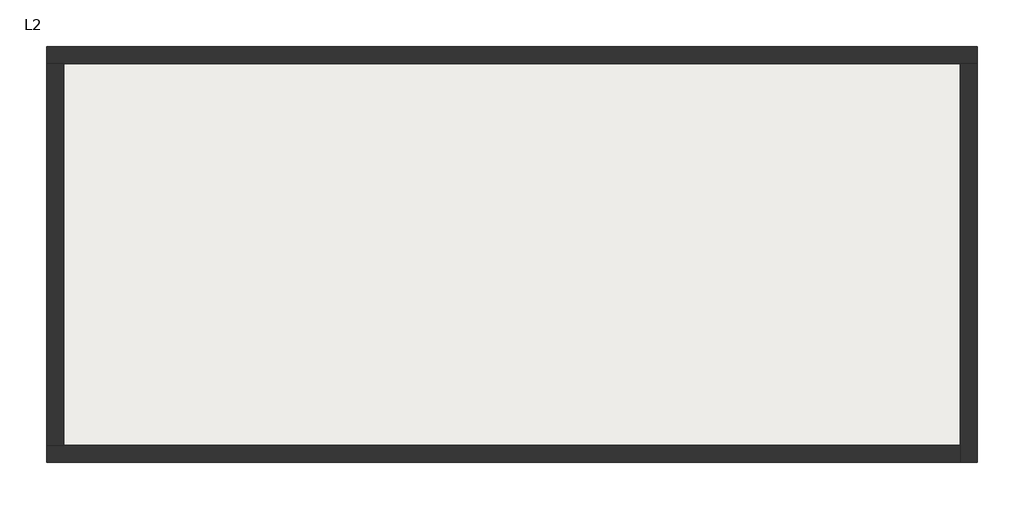
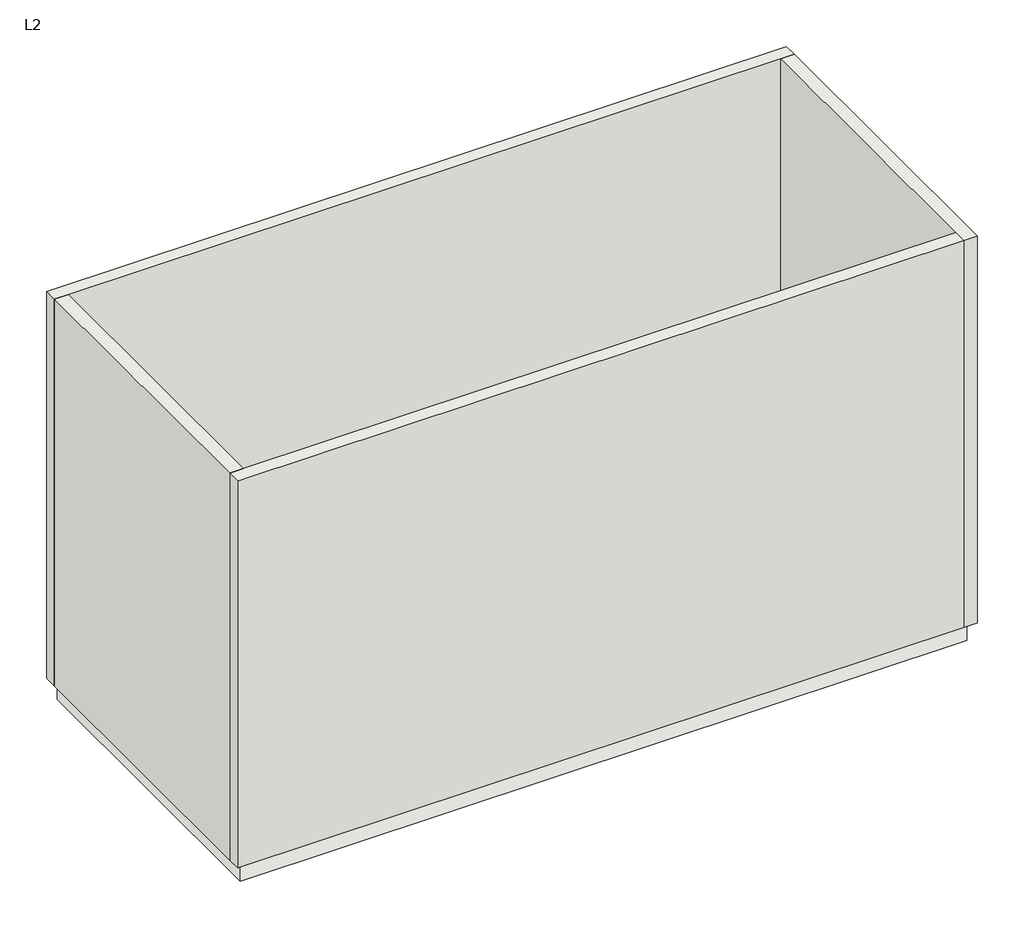
# One storey: 4 walls, 1 slab.
"""IFC4 building model written with IfcOpenShell, lengths in millimetres."""

import ifcopenshell
import ifcopenshell.guid

model = None  # the IFC model being written
_history = None  # IfcOwnerHistory: only IFC2X3 demands one
_inside = {}  # id of a spatial element -> (the spatial element, [elements in it])
_under = {}  # id of a project, library or spatial element -> (it, [spatial elements below it])
_declared = {}  # id of a project -> (the project, [libraries it declares])
_typed = {}  # id of a type object -> (the type object, [elements of that type])
_made_of = {}  # id of a material, layer set ... -> (it, [elements and type objects made of it])


def new_model(schema):
    """Start an empty IFC model of exactly this schema.

    Asked for "IFC4X3", IfcOpenShell would pick the latest addendum, in which some entities
    have other attributes; the version numbers below select the first issue.
    IFC2X3 requires an IfcOwnerHistory on every rooted entity: one is made here for all.
    """
    global model, _history
    if schema == "IFC4X3":
        model = ifcopenshell.file(schema_version=(4, 3, 0, 0))
    else:
        model = ifcopenshell.file(schema=schema)
    _inside.clear()
    _under.clear()
    _declared.clear()
    _typed.clear()
    _made_of.clear()
    _history = None
    if model.schema == "IFC2X3":
        org = make("IfcOrganization", Name="unknown")
        user = make(
            "IfcPersonAndOrganization",
            ThePerson=make("IfcPerson", FamilyName="unknown"),
            TheOrganization=org,
        )
        app = make(
            "IfcApplication",
            ApplicationDeveloper=org,
            Version="unknown",
            ApplicationFullName="unknown",
            ApplicationIdentifier="unknown",
        )
        _history = make(
            "IfcOwnerHistory",
            OwningUser=user,
            OwningApplication=app,
            ChangeAction="ADDED",
            CreationDate=0,
        )
    return model


def make(cls, **values):
    """One entity of the class cls with the attributes given. An attribute that is None is left unset."""
    return model.create_entity(
        cls, **{name: value for name, value in values.items() if value is not None}
    )


def rooted(cls, **values):
    """An entity with a GlobalId (a new one), such as an element, a storey or a relation."""
    return make(cls, GlobalId=ifcopenshell.guid.new(), OwnerHistory=_history, **values)


def si_unit(unit_type, name, prefix=None):
    """IfcSIUnit, for example si_unit("LENGTHUNIT", "METRE", prefix="MILLI")."""
    return make("IfcSIUnit", UnitType=unit_type, Prefix=prefix, Name=name)


def assignment(units):
    """IfcUnitAssignment: the units of a project."""
    return None if units is None else make("IfcUnitAssignment", Units=units)


def point(xyz):
    """IfcCartesianPoint."""
    return None if xyz is None else make("IfcCartesianPoint", Coordinates=xyz)


def direction(xyz):
    """IfcDirection."""
    return None if xyz is None else make("IfcDirection", DirectionRatios=xyz)


def frame(location, z_axis=None, x_axis=None):
    """IfcAxis2Placement3D, a coordinate frame: its origin and axes. An axis left out is left unset."""
    return make(
        "IfcAxis2Placement3D",
        Location=point(location),
        Axis=direction(z_axis),
        RefDirection=direction(x_axis),
    )


def origin():
    """The frame at (0, 0, 0) with its axes left unset."""
    return frame((0.0, 0.0, 0.0))


def place(relative_to, where):
    """IfcLocalPlacement: puts the frame where relative to a parent placement (None: the world)."""
    return make(
        "IfcLocalPlacement", PlacementRelTo=relative_to, RelativePlacement=where
    )


def context(
    kind, dimensions, precision=None, world=None, true_north=None, identifier=None
):
    """IfcGeometricRepresentationContext, for example the 3D "Model" context."""
    return make(
        "IfcGeometricRepresentationContext",
        ContextIdentifier=identifier,
        ContextType=kind,
        CoordinateSpaceDimension=dimensions,
        Precision=precision,
        WorldCoordinateSystem=world,
        TrueNorth=true_north,
    )


def project(units=None, contexts=None):
    """IfcProject with its units and contexts."""
    return rooted(
        "IfcProject",
        Name="project",
        RepresentationContexts=contexts,
        UnitsInContext=assignment(units),
    )


def spatial(cls, under=None, at=None, **own):
    """A site, building, storey or space (cls), placed at a placement, below another one or the project."""
    s = rooted(cls, ObjectPlacement=at, **own)
    if under is not None:
        _under.setdefault(under.id(), (under, []))[1].append(s)
    return s


def polyline(points):
    """IfcPolyline through the points."""
    return make("IfcPolyline", Points=[point(p) for p in points])


def outline(outer, holes=None, kind="AREA"):
    """IfcArbitraryClosedProfileDef: a profile drawn as a closed curve; with holes, ...WithVoids."""
    if holes is None:
        return make("IfcArbitraryClosedProfileDef", ProfileType=kind, OuterCurve=outer)
    return make(
        "IfcArbitraryProfileDefWithVoids",
        ProfileType=kind,
        OuterCurve=outer,
        InnerCurves=holes,
    )


def extrude(swept, where, along, depth):
    """IfcExtrudedAreaSolid: the profile swept, set in the frame where, extruded along a direction by depth."""
    return make(
        "IfcExtrudedAreaSolid",
        SweptArea=swept,
        Position=where,
        ExtrudedDirection=direction(along),
        Depth=depth,
    )


def faces_of(points, faces, orient=None, outer=None):
    """IfcFace entities. A face is a list of loops; a loop is a list of indices into points, from 0.

    orient and outer hold one flag for each loop. By default every Orientation is true, the
    first loop of a face is its IfcFaceOuterBound and the others are IfcFaceBound.
    """
    made = []
    for i, loops in enumerate(faces):
        bounds = []
        for j, loop in enumerate(loops):
            is_outer = j == 0 if outer is None else outer[i][j]
            bounds.append(
                make(
                    "IfcFaceOuterBound" if is_outer else "IfcFaceBound",
                    Bound=make("IfcPolyLoop", Polygon=[points[k] for k in loop]),
                    Orientation=True if orient is None else orient[i][j],
                )
            )
        made.append(make("IfcFace", Bounds=bounds))
    return made


def faceted_brep(points, faces, orient=None, outer=None, voids=None):
    """IfcFacetedBrep: a solid bounded by flat faces; with voids (closed shells), ...WithVoids."""
    shared = [point(p) for p in points]
    hull = make("IfcClosedShell", CfsFaces=faces_of(shared, faces, orient, outer))
    if voids is None:
        return make("IfcFacetedBrep", Outer=hull)
    return make(
        "IfcFacetedBrepWithVoids",
        Outer=hull,
        Voids=[
            make(cls, CfsFaces=faces_of(shared, fs, o, b)) for cls, fs, o, b in voids
        ],
    )


def shape(context_of_items, identifier, shape_type, items):
    """IfcShapeRepresentation: the items that make up one representation, for example the "Body"."""
    return make(
        "IfcShapeRepresentation",
        ContextOfItems=context_of_items,
        RepresentationIdentifier=identifier,
        RepresentationType=shape_type,
        Items=items,
    )


def made_of(thing, what):
    """Note that an element or type object is made of a material, layer set ...; save() writes the relation."""
    if what is not None:
        _made_of.setdefault(what.id(), (what, []))[1].append(thing)
    return thing


def element(
    cls,
    number,
    at=None,
    inside=None,
    cuts=None,
    type_object=None,
    material=None,
    context=None,
    identifier="Body",
    shape_type=None,
    held_by="IfcProductDefinitionShape",
    body=None,
    shapes=None,
    **own,
):
    """One element of the class cls, such as IfcWall. Its Tag is "e" and its number.

    at: its placement. inside: the storey or other place that contains it. cuts: it is an
    opening in that element (IfcRelVoidsElement). A single representation is given by context,
    identifier, shape_type and body (its items); several are given by shapes. held_by: the class
    of the entity that holds the representations. save() writes the other relations.
    """
    e = rooted(cls, Tag="e%d" % number, ObjectPlacement=at, **own)
    if body is not None:
        shapes = [shape(context, identifier, shape_type, body)]
    if shapes is not None:
        e.Representation = make(held_by, Representations=shapes)
    if inside is not None:
        _inside.setdefault(inside.id(), (inside, []))[1].append(e)
    if cuts is not None:
        rooted(
            "IfcRelVoidsElement", RelatingBuildingElement=cuts, RelatedOpeningElement=e
        )
    if type_object is not None:
        _typed.setdefault(type_object.id(), (type_object, []))[1].append(e)
    return made_of(e, material)


def aggregate(whole, parts):
    """IfcRelAggregates: a whole, such as a stair, and the parts it consists of."""
    return rooted("IfcRelAggregates", RelatingObject=whole, RelatedObjects=parts)


def save(model, path):
    """Write the relations noted so far, then the file.

    IfcRelAggregates (storeys below a building ...), IfcRelContainedInSpatialStructure (elements
    in a storey), IfcRelDefinesByType, IfcRelAssociatesMaterial and IfcRelDeclares: one each for
    every whole, place, type object, material and project.
    """
    for whole, parts in _under.values():
        aggregate(whole, parts)
    for where, things in _inside.values():
        rooted(
            "IfcRelContainedInSpatialStructure",
            RelatedElements=things,
            RelatingStructure=where,
        )
    for kind, things in _typed.values():
        rooted("IfcRelDefinesByType", RelatedObjects=things, RelatingType=kind)
    for what, things in _made_of.values():
        rooted("IfcRelAssociatesMaterial", RelatedObjects=things, RelatingMaterial=what)
    for by, libraries in _declared.values():
        rooted("IfcRelDeclares", RelatingContext=by, RelatedDefinitions=libraries)
    model.write(path)


model = new_model("IFC4")

# Units and contexts
model_context = context("Model", 3, world=origin())
ifc_project = project(units=[si_unit("LENGTHUNIT", "METRE", prefix="MILLI")], contexts=[model_context])

# Site, building, storey
site = spatial("IfcSite", under=ifc_project)
building = spatial("IfcBuilding", under=site)
storey = spatial("IfcBuildingStorey", under=building, Name="L2", Elevation=3657.6)

# Slab
placement = place(None, origin())
element("IfcSlab", 1, ObjectType="Generic - 12\"", at=placement, inside=storey, context=model_context, shape_type="SweptSolid", body=[
    extrude(outline(polyline([(23729.8135056, 3861.9420889), (12909.4135056, 3861.9420889), (12909.4135056, 8586.3420889), (23729.8135056, 8586.3420889), (23729.8135056, 3861.9420889)])), frame((0.0, 0.0, 3352.8), z_axis=(0.0, 0.0, 1.0), x_axis=(1.0, 0.0, 0.0)), (0.0, 0.0, 1.0), 304.8),
])

# Walls
element("IfcWall", 2, ObjectType="Generic - 8\"", at=placement, inside=storey, context=model_context, shape_type="Brep", body=[
    faceted_brep([(23831.4135056, 8687.9420889, 3657.6), (12807.8135056, 8687.9420889, 3657.6), (12807.8135056, 8687.9420889, 9753.6), (23831.4135056, 8687.9420889, 9753.6), (23831.4135056, 8484.7420889, 3657.6), (23831.4135056, 8484.7420889, 9753.6), (23628.2135056, 8484.7420889, 9753.6), (13011.0135056, 8484.7420889, 9753.6), (12807.8135056, 8484.7420889, 9753.6), (12807.8135056, 8484.7420889, 3657.6), (13011.0135056, 8484.7420889, 3657.6), (23628.2135056, 8484.7420889, 3657.6)], [[[0, 1, 2, 3]], [[4, 5, 6, 7, 8, 9, 10, 11]], [[1, 0, 4, 11, 10, 9]], [[3, 2, 8, 7, 6, 5]], [[0, 3, 5, 4]], [[2, 1, 9, 8]]]),
])
element("IfcWall", 3, ObjectType="Generic - 8\"", at=placement, inside=storey, context=model_context, shape_type="Brep", body=[
    faceted_brep([(23831.4135056, 3760.3420889, 3657.6), (23831.4135056, 8484.7420889, 3657.6), (23831.4135056, 8484.7420889, 9753.6), (23831.4135056, 3760.3420889, 9753.6), (23628.2135056, 3760.3420889, 3657.6), (23628.2135056, 3760.3420889, 9753.6), (23628.2135056, 3963.5420889, 9753.6), (23628.2135056, 8484.7420889, 9753.6), (23628.2135056, 8484.7420889, 3657.6), (23628.2135056, 3963.5420889, 3657.6)], [[[0, 1, 2, 3]], [[4, 5, 6, 7, 8, 9]], [[1, 0, 4, 9, 8]], [[3, 2, 7, 6, 5]], [[2, 1, 8, 7]], [[0, 3, 5, 4]]]),
])
element("IfcWall", 4, ObjectType="Generic - 8\"", at=placement, inside=storey, context=model_context, shape_type="Brep", body=[
    faceted_brep([(12807.8135056, 3760.3420889, 3657.6), (23628.2135056, 3760.3420889, 3657.6), (23628.2135056, 3760.3420889, 9753.6), (12807.8135056, 3760.3420889, 9753.6), (12807.8135056, 3963.5420889, 3657.6), (12807.8135056, 3963.5420889, 9753.6), (13011.0135056, 3963.5420889, 9753.6), (23628.2135056, 3963.5420889, 9753.6), (23628.2135056, 3963.5420889, 3657.6), (13011.0135056, 3963.5420889, 3657.6)], [[[0, 1, 2, 3]], [[4, 5, 6, 7, 8, 9]], [[1, 0, 4, 9, 8]], [[3, 2, 7, 6, 5]], [[2, 1, 8, 7]], [[0, 3, 5, 4]]]),
])
element("IfcWall", 5, ObjectType="Generic - 8\"", at=placement, inside=storey, context=model_context, shape_type="SweptSolid", body=[
    extrude(outline(polyline([(12807.8135056, 3963.5420889), (12807.8135056, 8484.7420889), (13011.0135056, 8484.7420889), (13011.0135056, 3963.5420889), (12807.8135056, 3963.5420889)])), frame((0.0, 0.0, 3657.6), z_axis=(0.0, 0.0, 1.0), x_axis=(1.0, 0.0, 0.0)), (0.0, 0.0, 1.0), 6096.0),
])

save(model, "model.ifc")

# Revit data of these elements
# Project information
#   Organization Name = "Organization Name"
#   Organization Description = "Organization Description"
#   Building Name = "Building Name"
#   Project Issue Date = "Issue Date"
#   Project Status = "Project Status"
#   Client Name = "Client Name"
#   Project Address = "Enter address here\nAddress Line 2"
#   Project Name = "Project Name"
#   Project Number = "Project Number"
# Type "Generic - 12\""
#   Description = "Generic Floor (Material By Category), 12\" thick"
#   Type Mark = "G01"
#   Function = 0
#   Layers, outside or top first: 1' - 0" no material (function 1)
# Type "Generic - 8\""
#   Description = "Generic Wall (Material By Category), 8\" thick"
#   Type Mark = "G06"
#   Layers, outside or top first: 0' - 8" no material (function 1)
# Element 1 (IfcSlab, "Generic - 12\"")
#   Height Offset From Level = 0' - 0"
#   Phase Created = New Construction
#   Materials on its faces: "Default Floor"
# Elements 2, 3, 4, 5 (IfcWall, "Generic - 8\"")
#   Top Offset = 0' - 0"
#   Base Offset = 0' - 0"
#   Unconnected Height = 20' - 0"
#   wall height = 20' - 0"
#   Phase Created = New Construction
#   Base Constraint = L2
#   Materials on its faces: "Default Wall"
# Materials
#   "Default Floor": class "Miscellaneous", colour RGB 128 128 128, transparency 0, Cost = 0
#   "Default Wall": class "Miscellaneous", colour RGB 192 192 192, transparency 0, Cost = 0
